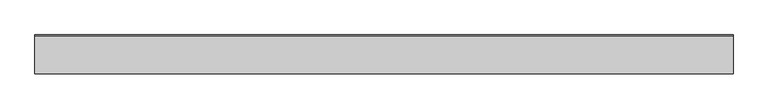
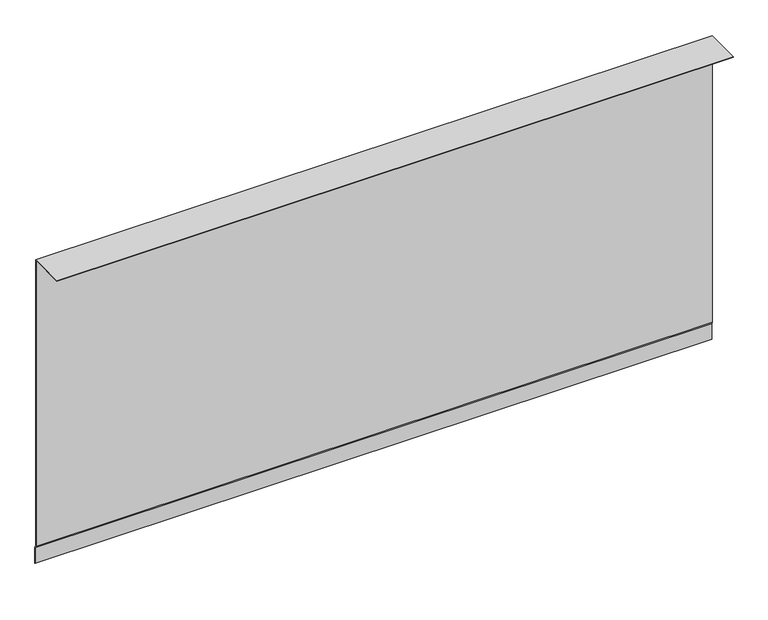
"""IFC4 building model written with IfcOpenShell, lengths in millimetres: proxy geometry, Membrane003 1195 : Membrane003 1195."""

from ifc_helpers import new_model, si_unit, frame, origin, place, context, project, spatial, polyline, outline, extrude, source, transform, mapped, element, save


def generic_models_7f0a8db5(model_context):
    return source(origin(), model_context, "Body", "SweptSolid", [
        extrude(outline(polyline([(9754.8834401, 36597.8828125), (9750.723729, 36604.890625), (9750.723729, 37497.8101563), (9644.9242604, 37497.8101563), (9644.9242604, 37499.3101563), (9752.223729, 37499.3101563), (9752.223729, 36605.3022818), (9756.3834401, 36598.2944693), (9756.3834401, 36548.0898438), (9754.8834401, 36548.0898438), (9754.8834401, 36597.8828125)])), frame((3694.2883192, 0.0, 0.0), z_axis=(1.0, 0.0, 0.0), x_axis=(0.0, 1.0, 0.0)), (0.0, 0.0, 1.0), 2000.0),
    ])


if __name__ == "__main__":
    model = new_model("IFC4")
    model_context = context("Model", 3, world=origin())
    ifc_project = project(units=[si_unit("LENGTHUNIT", "METRE", prefix="MILLI")], contexts=[model_context])
    site = spatial("IfcSite", under=ifc_project)
    building = spatial("IfcBuilding", under=site)
    placement = place(None, origin())
    generic_models_shape = generic_models_7f0a8db5(model_context)
    element("IfcBuildingElementProxy", 1, Name="Membrane003 1195 : Membrane003 1195", ObjectType="Membrane003 1195 : Membrane003 1195", at=placement, inside=building, context=model_context, shape_type="MappedRepresentation", body=[
        mapped(generic_models_shape, transform((0.0, 0.0, 0.0), x_axis=(1.0, 0.0, 0.0), y_axis=(0.0, 1.0, 0.0), z_axis=(0.0, 0.0, 1.0))),
    ])
    save(model, "model.ifc")

# Revit data of these elements
# Type "Membrane003 1195 : Membrane003 1195"
#   NameOverride = "Membrane003"
# Element 1 (IfcBuildingElementProxy, "Membrane003 1195 : Membrane003 1195")
#   Materials on its faces: "2 LAYERS NO. 30 ASTM D226 ASPHALT SATURATED ORGANIC FELT"
# Materials
#   "2 LAYERS NO. 30 ASTM D226 ASPHALT SATURATED ORGANIC FELT": class "Unassigned", colour RGB 46 171 0, transparency 0
